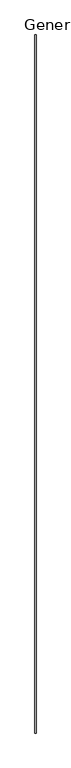
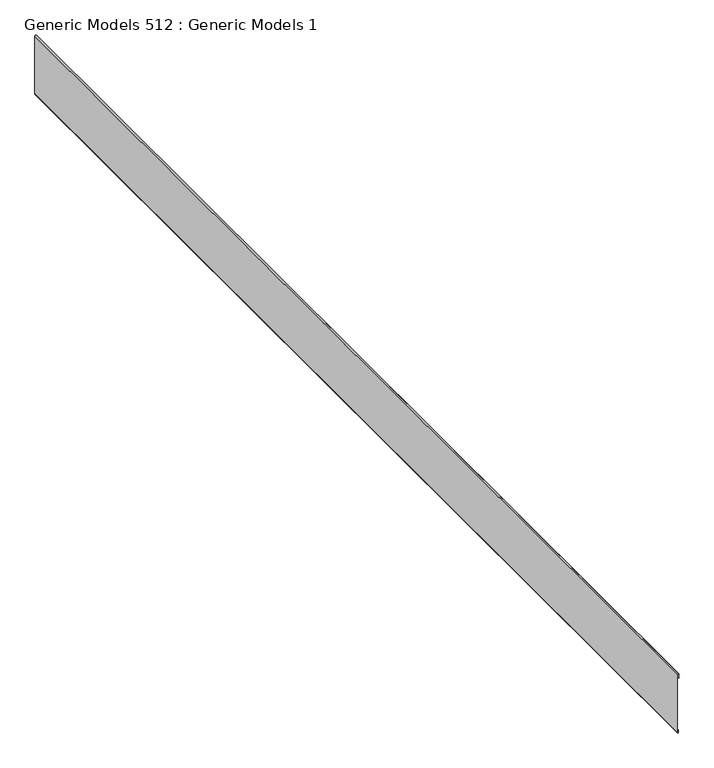
"""IFC4 building model written with IfcOpenShell, lengths in millimetres: proxy geometry, Generic Models 512 : Generic Models 1."""

from ifc_helpers import new_model, si_unit, point, frame, frame_2d, origin, place, context, project, spatial, polyline, circle_curve, trimmed, segment, composite_curve, outline, extrude, source, transform, mapped, element, save


def generic_models_512_generic_models_1_b77a654e(model_context):
    return source(origin(), model_context, "Body", "SweptSolid", [
        extrude(outline(composite_curve([segment(polyline([(129830.907875, -7140.4961539), (129846.1600973, -7140.4961539), (129846.1600973, -7142.0836539), (129830.907875, -7142.0836539)]), True, "CONTINUOUS"), segment(trimmed(circle_curve(frame_2d((129830.907875, -7144.1699111)), 2.0862572), [point((129830.907875, -7142.0836539))], [point((129830.907875, -7146.2561683))], True, "CARTESIAN"), True, "CONTINUOUS"), segment(polyline([(129830.907875, -7146.2561683), (130191.0914609, -7146.2561683)]), True, "CONTINUOUS"), segment(trimmed(circle_curve(frame_2d((130191.0914609, -7142.3839736)), 3.8721947), [point((130191.0914609, -7146.2561683))], [point((130191.0914609, -7138.5117789))], True, "CARTESIAN"), True, "CONTINUOUS"), segment(polyline([(130191.0914609, -7138.5117789), (130165.9173635, -7138.5117789), (130165.9173635, -7136.9242789), (130191.0914609, -7136.9242789)]), True, "CONTINUOUS"), segment(trimmed(circle_curve(frame_2d((130191.0914609, -7142.3839736)), 5.4596947), [point((130191.0914609, -7136.9242789))], [point((130191.0914609, -7147.8436683))], False, "CARTESIAN"), True, "CONTINUOUS"), segment(polyline([(130191.0914609, -7147.8436683), (129830.907875, -7147.8436683)]), True, "CONTINUOUS"), segment(trimmed(circle_curve(frame_2d((129830.907875, -7144.1699111)), 3.6737572), [point((129830.907875, -7147.8436683))], [point((129830.907875, -7140.4961539))], False, "CARTESIAN"), True, "CONTINUOUS")], self_intersect=False)), frame((0.0, -7039.3472918, 0.0), z_axis=(0.0, 1.0, 0.0), x_axis=(0.0, 0.0, 1.0)), (0.0, 0.0, 1.0), 6575.224258),
    ])


if __name__ == "__main__":
    model = new_model("IFC4")
    model_context = context("Model", 3, world=origin())
    ifc_project = project(units=[si_unit("LENGTHUNIT", "METRE", prefix="MILLI")], contexts=[model_context])
    site = spatial("IfcSite", under=ifc_project)
    building = spatial("IfcBuilding", under=site)
    placement = place(None, origin())
    generic_models_512_generic_models_1_shape = generic_models_512_generic_models_1_b77a654e(model_context)
    element("IfcBuildingElementProxy", 1, Name="Generic Models 512 : Generic Models 1", ObjectType="Generic Models 512 : Generic Models 1", at=placement, inside=building, context=model_context, shape_type="MappedRepresentation", body=[
        mapped(generic_models_512_generic_models_1_shape, transform((0.0, 0.0, 0.0), x_axis=(1.0, 0.0, 0.0), y_axis=(0.0, 1.0, 0.0), z_axis=(0.0, 0.0, 1.0))),
    ])
    save(model, "model.ifc")

# Revit data of these elements
# Element 1 (IfcBuildingElementProxy, "Generic Models 512 : Generic Models 1")
#   Materials on its faces: "_16 GA. COPPER BRAKE METAL FASCIA"
# Materials
#   "_16 GA. COPPER BRAKE METAL FASCIA": class "Generic", colour RGB 175 175 175, transparency 0, Cost = 0
